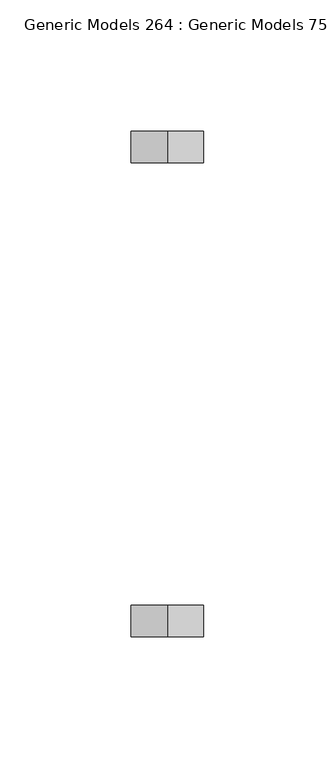
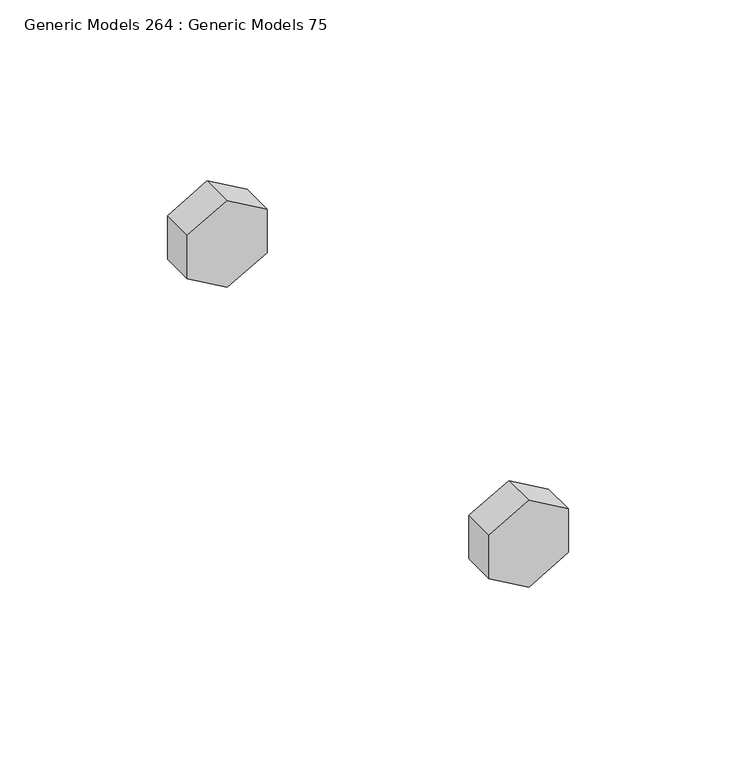
"""IFC4 building model written with IfcOpenShell, lengths in millimetres: proxy geometry, Generic Models 264 : Generic Models 75."""

from ifc_helpers import new_model, si_unit, frame, origin, place, context, project, spatial, polyline, outline, extrude, source, transform, mapped, element, save


def generic_models_264_generic_models_75_1e2ff585(model_context):
    return source(origin(), model_context, "Body", "SweptSolid", [
        extrude(outline(polyline([(268613.0902933, 31975.9942029), (268597.2537198, 31975.9942029), (268589.335433, 31989.7090778), (268597.2537198, 32003.4239528), (268613.0902933, 32003.4239528), (268621.00858, 31989.7090778), (268613.0902933, 31975.9942029)])), frame((0.0, 35373.9582942, 0.0), z_axis=(0.0, 1.0, 0.0), x_axis=(0.0, 0.0, 1.0)), (0.0, 0.0, 1.0), 11.90625),
        extrude(outline(polyline([(268613.0902933, 31975.9942029), (268597.2537198, 31975.9942029), (268589.335433, 31989.7090778), (268597.2537198, 32003.4239528), (268613.0902933, 32003.4239528), (268621.00858, 31989.7090778), (268613.0902933, 31975.9942029)])), frame((0.0, 35193.7770442, 0.0), z_axis=(0.0, 1.0, 0.0), x_axis=(0.0, 0.0, 1.0)), (0.0, 0.0, 1.0), 11.90625),
    ])


if __name__ == "__main__":
    model = new_model("IFC4")
    model_context = context("Model", 3, world=origin())
    ifc_project = project(units=[si_unit("LENGTHUNIT", "METRE", prefix="MILLI")], contexts=[model_context])
    site = spatial("IfcSite", under=ifc_project)
    building = spatial("IfcBuilding", under=site)
    placement = place(None, origin())
    generic_models_264_generic_models_75_shape = generic_models_264_generic_models_75_1e2ff585(model_context)
    element("IfcBuildingElementProxy", 1, Name="Generic Models 264 : Generic Models 75", ObjectType="Generic Models 264 : Generic Models 75", at=placement, inside=building, context=model_context, shape_type="MappedRepresentation", body=[
        mapped(generic_models_264_generic_models_75_shape, transform((0.0, 0.0, 0.0), x_axis=(1.0, 0.0, 0.0), y_axis=(0.0, 1.0, 0.0), z_axis=(0.0, 0.0, 1.0))),
    ])
    save(model, "model.ifc")

# Revit data of these elements
# Element 1 (IfcBuildingElementProxy, "Generic Models 264 : Generic Models 75")
#   Materials on its faces: "3/4\" GALV. THRU BOLTS"
# Materials
#   "3/4\" GALV. THRU BOLTS": class "Generic", colour RGB 105 69 171, transparency 0, Cost = 0
